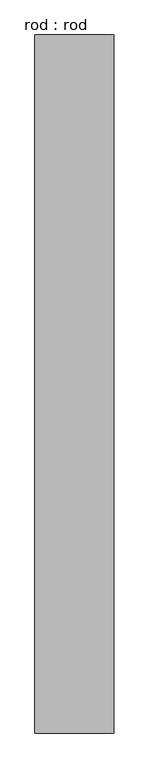
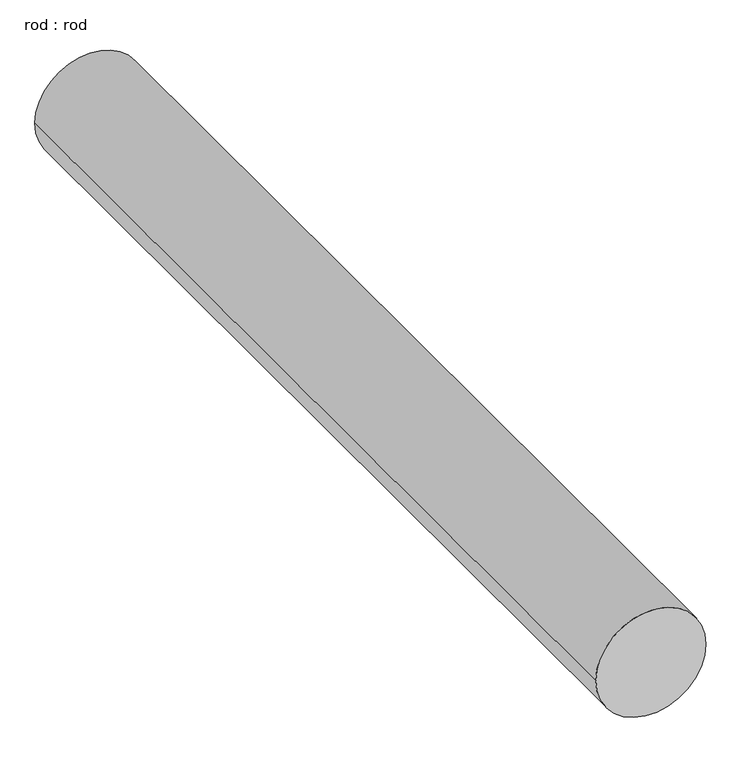
"""IFC4 building model written with IfcOpenShell, lengths in millimetres: proxy geometry, rod : rod."""

import ifcopenshell
import ifcopenshell.guid

model = None  # the IFC model being written
_history = None  # IfcOwnerHistory: only IFC2X3 demands one
_inside = {}  # id of a spatial element -> (the spatial element, [elements in it])
_under = {}  # id of a project, library or spatial element -> (it, [spatial elements below it])
_declared = {}  # id of a project -> (the project, [libraries it declares])
_typed = {}  # id of a type object -> (the type object, [elements of that type])
_made_of = {}  # id of a material, layer set ... -> (it, [elements and type objects made of it])


def new_model(schema):
    """Start an empty IFC model of exactly this schema.

    Asked for "IFC4X3", IfcOpenShell would pick the latest addendum, in which some entities
    have other attributes; the version numbers below select the first issue.
    IFC2X3 requires an IfcOwnerHistory on every rooted entity: one is made here for all.
    """
    global model, _history
    if schema == "IFC4X3":
        model = ifcopenshell.file(schema_version=(4, 3, 0, 0))
    else:
        model = ifcopenshell.file(schema=schema)
    _inside.clear()
    _under.clear()
    _declared.clear()
    _typed.clear()
    _made_of.clear()
    _history = None
    if model.schema == "IFC2X3":
        org = make("IfcOrganization", Name="unknown")
        user = make(
            "IfcPersonAndOrganization",
            ThePerson=make("IfcPerson", FamilyName="unknown"),
            TheOrganization=org,
        )
        app = make(
            "IfcApplication",
            ApplicationDeveloper=org,
            Version="unknown",
            ApplicationFullName="unknown",
            ApplicationIdentifier="unknown",
        )
        _history = make(
            "IfcOwnerHistory",
            OwningUser=user,
            OwningApplication=app,
            ChangeAction="ADDED",
            CreationDate=0,
        )
    return model


def make(cls, **values):
    """One entity of the class cls with the attributes given. An attribute that is None is left unset."""
    return model.create_entity(
        cls, **{name: value for name, value in values.items() if value is not None}
    )


def rooted(cls, **values):
    """An entity with a GlobalId (a new one), such as an element, a storey or a relation."""
    return make(cls, GlobalId=ifcopenshell.guid.new(), OwnerHistory=_history, **values)


def si_unit(unit_type, name, prefix=None):
    """IfcSIUnit, for example si_unit("LENGTHUNIT", "METRE", prefix="MILLI")."""
    return make("IfcSIUnit", UnitType=unit_type, Prefix=prefix, Name=name)


def assignment(units):
    """IfcUnitAssignment: the units of a project."""
    return None if units is None else make("IfcUnitAssignment", Units=units)


def point(xyz):
    """IfcCartesianPoint."""
    return None if xyz is None else make("IfcCartesianPoint", Coordinates=xyz)


def direction(xyz):
    """IfcDirection."""
    return None if xyz is None else make("IfcDirection", DirectionRatios=xyz)


def frame(location, z_axis=None, x_axis=None):
    """IfcAxis2Placement3D, a coordinate frame: its origin and axes. An axis left out is left unset."""
    return make(
        "IfcAxis2Placement3D",
        Location=point(location),
        Axis=direction(z_axis),
        RefDirection=direction(x_axis),
    )


def frame_2d(location, x_axis=None):
    """IfcAxis2Placement2D, a coordinate frame in the plane: its origin and x axis."""
    return make(
        "IfcAxis2Placement2D", Location=point(location), RefDirection=direction(x_axis)
    )


def origin():
    """The frame at (0, 0, 0) with its axes left unset."""
    return frame((0.0, 0.0, 0.0))


def place(relative_to, where):
    """IfcLocalPlacement: puts the frame where relative to a parent placement (None: the world)."""
    return make(
        "IfcLocalPlacement", PlacementRelTo=relative_to, RelativePlacement=where
    )


def context(
    kind, dimensions, precision=None, world=None, true_north=None, identifier=None
):
    """IfcGeometricRepresentationContext, for example the 3D "Model" context."""
    return make(
        "IfcGeometricRepresentationContext",
        ContextIdentifier=identifier,
        ContextType=kind,
        CoordinateSpaceDimension=dimensions,
        Precision=precision,
        WorldCoordinateSystem=world,
        TrueNorth=true_north,
    )


def project(units=None, contexts=None):
    """IfcProject with its units and contexts."""
    return rooted(
        "IfcProject",
        Name="project",
        RepresentationContexts=contexts,
        UnitsInContext=assignment(units),
    )


def spatial(cls, under=None, at=None, **own):
    """A site, building, storey or space (cls), placed at a placement, below another one or the project."""
    s = rooted(cls, ObjectPlacement=at, **own)
    if under is not None:
        _under.setdefault(under.id(), (under, []))[1].append(s)
    return s


def circle_curve(where, radius):
    """IfcCircle in the frame where."""
    return make("IfcCircle", Position=where, Radius=radius)


def trimmed(basis, trim1, trim2, sense, master):
    """IfcTrimmedCurve: the piece of a basis curve between two trims."""
    return make(
        "IfcTrimmedCurve",
        BasisCurve=basis,
        Trim1=trim1,
        Trim2=trim2,
        SenseAgreement=sense,
        MasterRepresentation=master,
    )


def segment(curve, same_sense, transition):
    """IfcCompositeCurveSegment."""
    return make(
        "IfcCompositeCurveSegment",
        Transition=transition,
        SameSense=same_sense,
        ParentCurve=curve,
    )


def composite_curve(segments, self_intersect=None):
    """IfcCompositeCurve: segments joined end to end."""
    return make("IfcCompositeCurve", Segments=segments, SelfIntersect=self_intersect)


def outline(outer, holes=None, kind="AREA"):
    """IfcArbitraryClosedProfileDef: a profile drawn as a closed curve; with holes, ...WithVoids."""
    if holes is None:
        return make("IfcArbitraryClosedProfileDef", ProfileType=kind, OuterCurve=outer)
    return make(
        "IfcArbitraryProfileDefWithVoids",
        ProfileType=kind,
        OuterCurve=outer,
        InnerCurves=holes,
    )


def extrude(swept, where, along, depth):
    """IfcExtrudedAreaSolid: the profile swept, set in the frame where, extruded along a direction by depth."""
    return make(
        "IfcExtrudedAreaSolid",
        SweptArea=swept,
        Position=where,
        ExtrudedDirection=direction(along),
        Depth=depth,
    )


def shape(context_of_items, identifier, shape_type, items):
    """IfcShapeRepresentation: the items that make up one representation, for example the "Body"."""
    return make(
        "IfcShapeRepresentation",
        ContextOfItems=context_of_items,
        RepresentationIdentifier=identifier,
        RepresentationType=shape_type,
        Items=items,
    )


def source(mapping_origin, context_of_items, identifier, shape_type, items):
    """IfcRepresentationMap: a shape defined once, which mapped items show again and again."""
    return make(
        "IfcRepresentationMap",
        MappingOrigin=mapping_origin,
        MappedRepresentation=shape(context_of_items, identifier, shape_type, items),
    )


def transform(
    local_origin,
    x_axis=None,
    y_axis=None,
    z_axis=None,
    scale=None,
    scale2=None,
    scale3=None,
    uniform=True,
):
    """IfcCartesianTransformationOperator3D, or its non-uniform kind. x_axis, y_axis, z_axis: its Axis1, 2, 3."""
    if uniform:
        return make(
            "IfcCartesianTransformationOperator3D",
            Axis1=direction(x_axis),
            Axis2=direction(y_axis),
            LocalOrigin=point(local_origin),
            Scale=scale,
            Axis3=direction(z_axis),
        )
    return make(
        "IfcCartesianTransformationOperator3DnonUniform",
        Axis1=direction(x_axis),
        Axis2=direction(y_axis),
        LocalOrigin=point(local_origin),
        Scale=scale,
        Axis3=direction(z_axis),
        Scale2=scale2,
        Scale3=scale3,
    )


def mapped(mapping_source, mapping_target):
    """IfcMappedItem: shows the shape of a source again, moved by a transform."""
    return make(
        "IfcMappedItem", MappingSource=mapping_source, MappingTarget=mapping_target
    )


def made_of(thing, what):
    """Note that an element or type object is made of a material, layer set ...; save() writes the relation."""
    if what is not None:
        _made_of.setdefault(what.id(), (what, []))[1].append(thing)
    return thing


def element(
    cls,
    number,
    at=None,
    inside=None,
    cuts=None,
    type_object=None,
    material=None,
    context=None,
    identifier="Body",
    shape_type=None,
    held_by="IfcProductDefinitionShape",
    body=None,
    shapes=None,
    **own,
):
    """One element of the class cls, such as IfcWall. Its Tag is "e" and its number.

    at: its placement. inside: the storey or other place that contains it. cuts: it is an
    opening in that element (IfcRelVoidsElement). A single representation is given by context,
    identifier, shape_type and body (its items); several are given by shapes. held_by: the class
    of the entity that holds the representations. save() writes the other relations.
    """
    e = rooted(cls, Tag="e%d" % number, ObjectPlacement=at, **own)
    if body is not None:
        shapes = [shape(context, identifier, shape_type, body)]
    if shapes is not None:
        e.Representation = make(held_by, Representations=shapes)
    if inside is not None:
        _inside.setdefault(inside.id(), (inside, []))[1].append(e)
    if cuts is not None:
        rooted(
            "IfcRelVoidsElement", RelatingBuildingElement=cuts, RelatedOpeningElement=e
        )
    if type_object is not None:
        _typed.setdefault(type_object.id(), (type_object, []))[1].append(e)
    return made_of(e, material)


def aggregate(whole, parts):
    """IfcRelAggregates: a whole, such as a stair, and the parts it consists of."""
    return rooted("IfcRelAggregates", RelatingObject=whole, RelatedObjects=parts)


def save(model, path):
    """Write the relations noted so far, then the file.

    IfcRelAggregates (storeys below a building ...), IfcRelContainedInSpatialStructure (elements
    in a storey), IfcRelDefinesByType, IfcRelAssociatesMaterial and IfcRelDeclares: one each for
    every whole, place, type object, material and project.
    """
    for whole, parts in _under.values():
        aggregate(whole, parts)
    for where, things in _inside.values():
        rooted(
            "IfcRelContainedInSpatialStructure",
            RelatedElements=things,
            RelatingStructure=where,
        )
    for kind, things in _typed.values():
        rooted("IfcRelDefinesByType", RelatedObjects=things, RelatingType=kind)
    for what, things in _made_of.values():
        rooted("IfcRelAssociatesMaterial", RelatedObjects=things, RelatingMaterial=what)
    for by, libraries in _declared.values():
        rooted("IfcRelDeclares", RelatingContext=by, RelatedDefinitions=libraries)
    model.write(path)


def rod_rod_fa92ec96(model_context):
    return source(origin(), model_context, "Body", "SweptSolid", [
        extrude(outline(composite_curve([segment(trimmed(circle_curve(frame_2d((0.0108462, 0.0)), 200.0), [point((0.0108462, 200.0))], [point((0.0108462, -200.0))], False, "CARTESIAN"), True, "CONTINUOUS"), segment(trimmed(circle_curve(frame_2d((0.0108462, 0.0)), 200.0), [point((0.0108462, -200.0))], [point((0.0108462, 200.0))], False, "CARTESIAN"), True, "CONTINUOUS")], self_intersect=False)), frame((0.0, 2325.0871783, 0.0), z_axis=(0.0, 1.0, 0.0), x_axis=(0.0, 0.0, 1.0)), (0.0, 0.0, 1.0), 3535.2828741),
    ])


if __name__ == "__main__":
    model = new_model("IFC4")
    model_context = context("Model", 3, world=origin())
    ifc_project = project(units=[si_unit("LENGTHUNIT", "METRE", prefix="MILLI")], contexts=[model_context])
    site = spatial("IfcSite", under=ifc_project)
    building = spatial("IfcBuilding", under=site)
    placement = place(None, origin())
    rod_rod_shape = rod_rod_fa92ec96(model_context)
    element("IfcBuildingElementProxy", 1, Name="rod : rod", ObjectType="rod : rod", at=placement, inside=building, context=model_context, shape_type="MappedRepresentation", body=[
        mapped(rod_rod_shape, transform((0.0, 0.0, 0.0), x_axis=(1.0, 0.0, 0.0), y_axis=(0.0, 1.0, 0.0), z_axis=(0.0, 0.0, 1.0))),
    ])
    save(model, "model.ifc")

# Revit data of these elements
# Type "rod : rod"
#   Default Elevation = 0
